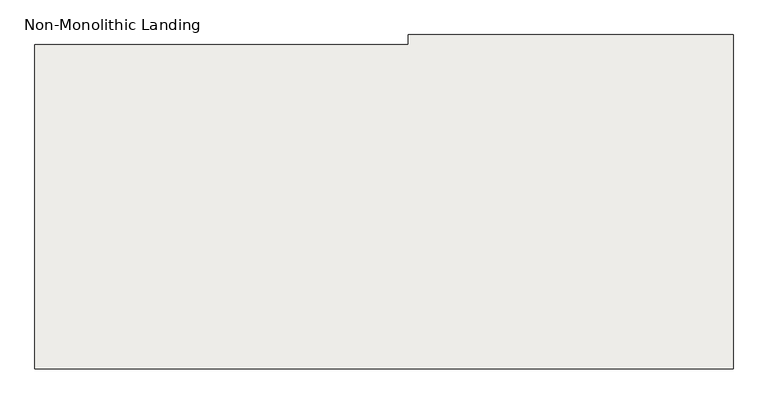
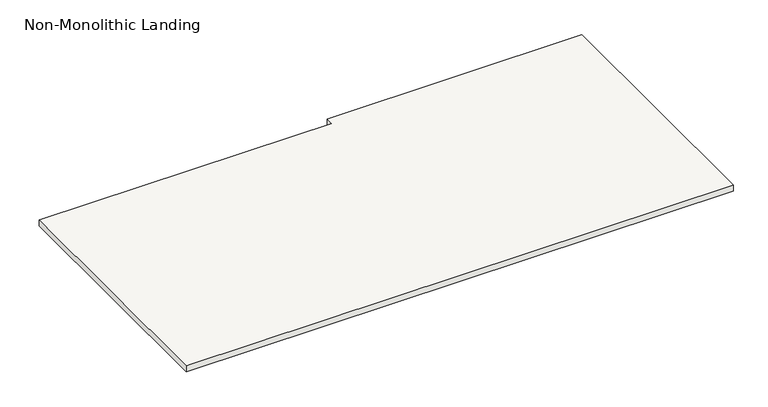
"""IFC4 building model written with IfcOpenShell, lengths in millimetres: slab geometry, Non-Monolithic Landing."""

from ifc_helpers import new_model, si_unit, frame, origin, place, context, project, spatial, polyline, outline, extrude, source, transform, mapped, element, save


def non_monolithic_landing_8f9c0fde(model_context):
    return source(origin(), model_context, "Body", "SweptSolid", [
        extrude(outline(polyline([(17000.0002442, 21429.9999999), (17000.0002442, 19369.9999999), (12700.0002443, 19369.9999999), (12700.0002443, 21369.9999999), (14700.0002443, 21369.9999999), (15000.0002442, 21369.9999999), (15000.0002442, 21429.9999999), (17000.0002442, 21429.9999999)])), frame((0.0, 0.0, 29116.6666667), z_axis=(0.0, 0.0, 1.0), x_axis=(1.0, 0.0, 0.0)), (0.0, 0.0, 1.0), 50.0),
    ])


if __name__ == "__main__":
    model = new_model("IFC4")
    model_context = context("Model", 3, world=origin())
    ifc_project = project(units=[si_unit("LENGTHUNIT", "METRE", prefix="MILLI")], contexts=[model_context])
    site = spatial("IfcSite", under=ifc_project)
    building = spatial("IfcBuilding", under=site)
    placement = place(None, origin())
    non_monolithic_landing_shape = non_monolithic_landing_8f9c0fde(model_context)
    element("IfcSlab", 1, ObjectType="Non-Monolithic Landing", at=placement, inside=building, context=model_context, shape_type="MappedRepresentation", body=[
        mapped(non_monolithic_landing_shape, transform((0.0, 0.0, 0.0), x_axis=(1.0, 0.0, 0.0), y_axis=(0.0, 1.0, 0.0), z_axis=(0.0, 0.0, 1.0))),
    ])
    save(model, "model.ifc")
